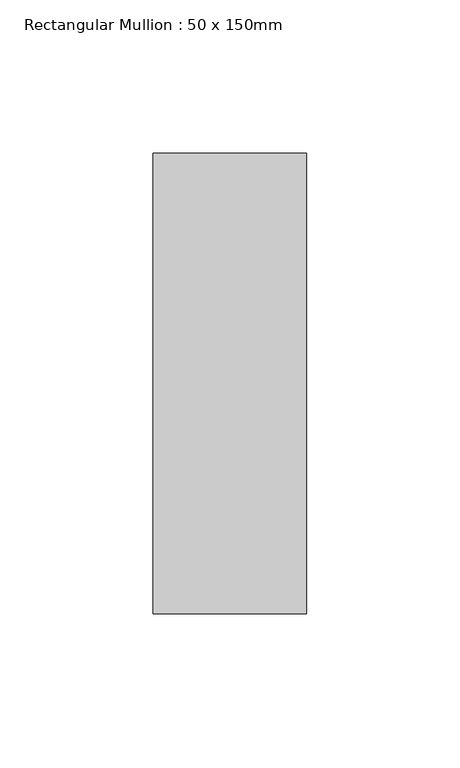
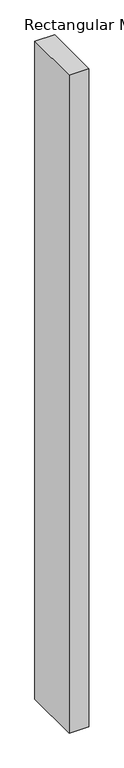
"""IFC4 building model written with IfcOpenShell, lengths in millimetres: member geometry, Rectangular Mullion : 50 x 150mm."""

from ifc_helpers import new_model, si_unit, frame, origin, place, context, project, spatial, polyline, outline, extrude, source, transform, mapped, element, save


def rectangular_mullion_50_x_150mm_661033a2(model_context):
    return source(origin(), model_context, "Body", "SweptSolid", [
        extrude(outline(polyline([(0.0, 75.0), (0.0, -75.0), (-50.0, -75.0), (-50.0, 75.0), (0.0, 75.0)])), frame((0.0, 0.0, -1759.0), z_axis=(0.0, 0.0, 1.0), x_axis=(1.0, 0.0, 0.0)), (0.0, 0.0, 1.0), 1759.0),
    ])


if __name__ == "__main__":
    model = new_model("IFC4")
    model_context = context("Model", 3, world=origin())
    ifc_project = project(units=[si_unit("LENGTHUNIT", "METRE", prefix="MILLI")], contexts=[model_context])
    site = spatial("IfcSite", under=ifc_project)
    building = spatial("IfcBuilding", under=site)
    placement = place(None, origin())
    rectangular_mullion_50_x_150mm_shape = rectangular_mullion_50_x_150mm_661033a2(model_context)
    element("IfcMember", 1, ObjectType="Rectangular Mullion : 50 x 150mm", at=placement, inside=building, context=model_context, shape_type="MappedRepresentation", body=[
        mapped(rectangular_mullion_50_x_150mm_shape, transform((0.0, 0.0, 0.0), x_axis=(1.0, 0.0, 0.0), y_axis=(0.0, 1.0, 0.0), z_axis=(0.0, 0.0, 1.0))),
    ])
    save(model, "model.ifc")

# Revit data of these elements
# Type "Rectangular Mullion : 50 x 150mm"
#   Keynote = "H11"
#   built-in parameter 1007304 = 0.492126 (stored number, unit not read)
#   built-in parameter 1007301 = 0.082021 (stored number, unit not read)
#   built-in parameter 1007300 = 0.082021 (stored number, unit not read)
# Element 1 (IfcMember, "Rectangular Mullion : 50 x 150mm")
#   Materials on its faces: "Aluminium"
# Materials
#   "Aluminium": class "Metal", colour RGB 247 247 247, transparency 0, Description = "Aluminium 6061", Cost = 0
